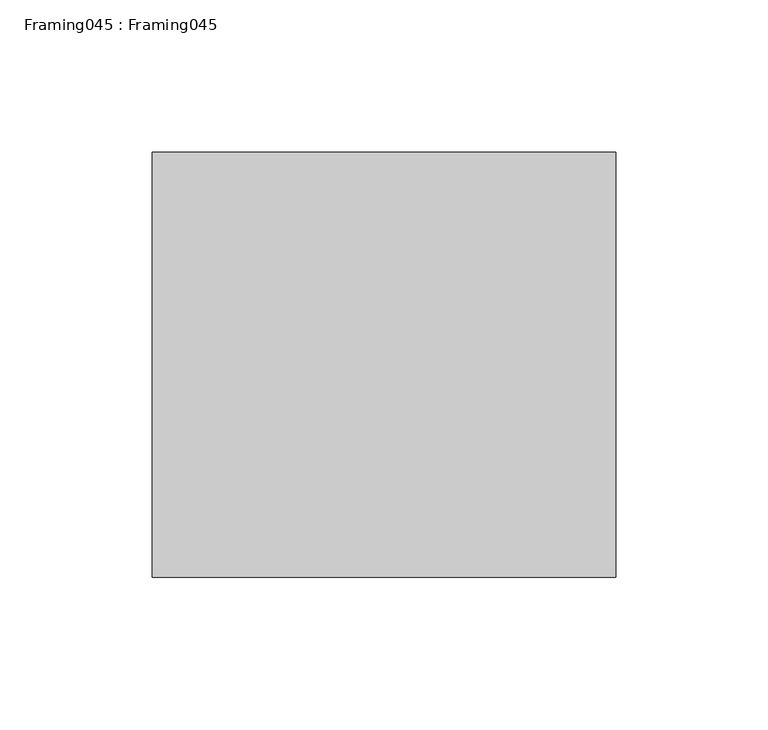
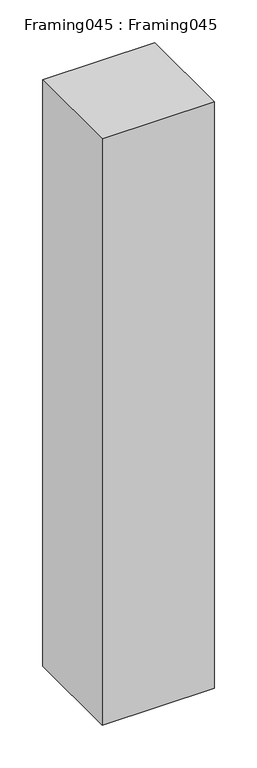
"""IFC4 building model written with IfcOpenShell, lengths in millimetres: proxy geometry, Framing045 : Framing045."""

from ifc_helpers import new_model, si_unit, frame, origin, place, context, project, spatial, polyline, outline, extrude, source, transform, mapped, element, save


def framing045_framing045_6d0a6c63(model_context):
    return source(origin(), model_context, "Body", "SweptSolid", [
        extrude(outline(polyline([(13687.8178845, -4250.1925368), (13687.8178845, -4389.8925368), (13535.4178845, -4389.8925368), (13535.4178845, -4250.1925368), (13687.8178845, -4250.1925368)])), frame((0.0, 0.0, 40163.496), z_axis=(0.0, 0.0, 1.0), x_axis=(1.0, 0.0, 0.0)), (0.0, 0.0, 1.0), 841.3827187),
    ])


if __name__ == "__main__":
    model = new_model("IFC4")
    model_context = context("Model", 3, world=origin())
    ifc_project = project(units=[si_unit("LENGTHUNIT", "METRE", prefix="MILLI")], contexts=[model_context])
    site = spatial("IfcSite", under=ifc_project)
    building = spatial("IfcBuilding", under=site)
    placement = place(None, origin())
    framing045_framing045_shape = framing045_framing045_6d0a6c63(model_context)
    element("IfcBuildingElementProxy", 1, Name="Framing045 : Framing045", ObjectType="Framing045 : Framing045", at=placement, inside=building, context=model_context, shape_type="MappedRepresentation", body=[
        mapped(framing045_framing045_shape, transform((0.0, 0.0, 0.0), x_axis=(1.0, 0.0, 0.0), y_axis=(0.0, 1.0, 0.0), z_axis=(0.0, 0.0, 1.0))),
    ])
    save(model, "model.ifc")

# Revit data of these elements
# Type "Framing045 : Framing045"
#   NameOverride = "Framing045"
# Element 1 (IfcBuildingElementProxy, "Framing045 : Framing045")
#   Materials on its faces: "WOOD FRAMING (SEE STRUCT DWGS)"
# Materials
#   "WOOD FRAMING (SEE STRUCT DWGS)": class "Unassigned", colour RGB 224 188 168, transparency 0, Cost = 0
